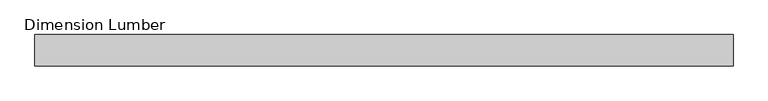
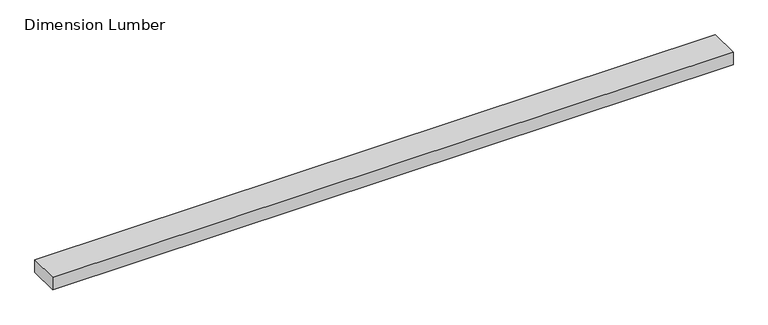
"""IFC4 building model written with IfcOpenShell, lengths in millimetres: beam geometry, Dimension Lumber : Top Supporting Lumbers."""

from ifc_helpers import new_model, si_unit, frame, origin, place, context, project, spatial, polyline, outline, extrude, source, transform, mapped, element, save


def dimension_lumber_b8718559(model_context):
    return source(origin(), model_context, "Body", "SweptSolid", [
        extrude(outline(polyline([(987.425, 44.45), (987.425, -44.45), (-987.425, -44.45), (-987.425, 44.45), (987.425, 44.45)])), frame((0.0, 0.0, -19.05), z_axis=(0.0, 0.0, 1.0), x_axis=(1.0, 0.0, 0.0)), (0.0, 0.0, 1.0), 38.1),
    ])


if __name__ == "__main__":
    model = new_model("IFC4")
    model_context = context("Model", 3, world=origin())
    ifc_project = project(units=[si_unit("LENGTHUNIT", "METRE", prefix="MILLI")], contexts=[model_context])
    site = spatial("IfcSite", under=ifc_project)
    building = spatial("IfcBuilding", under=site)
    placement = place(None, origin())
    dimension_lumber_shape = dimension_lumber_b8718559(model_context)
    element("IfcBeam", 1, ObjectType="Dimension Lumber : Top Supporting Lumbers", at=placement, inside=building, context=model_context, shape_type="MappedRepresentation", body=[
        mapped(dimension_lumber_shape, transform((0.0, 0.0, 0.0), x_axis=(1.0, 0.0, 0.0), y_axis=(0.0, 1.0, 0.0), z_axis=(0.0, 0.0, 1.0))),
    ])
    save(model, "model.ifc")

# Revit data of these elements
# Type "Dimension Lumber : Top Supporting Lumbers"
#   Assembly Code = "B10"
#   A = 0.0364583 SF
#   Length [instance default] = 5' - 0"
#   b = 0' - 3 1/2"
#   d = 0' - 1 1/2"
#   Structural Material [instance default] = Softwood, Lumber
# Element 1 (IfcBeam, "Dimension Lumber : Top Supporting Lumbers")
#   Structural Material = Douglas Fir #2
#   Materials on its faces: "Douglas Fir #2"
# Materials
#   "Softwood, Lumber": class "Wood", colour RGB 223 192 134, transparency 0, Description = "Pinus Echinata", Cost = 0
#   "Douglas Fir #2": class "Wood", colour RGB 223 192 134, transparency 0, Description = "Pinus Echinata", Cost = 0
